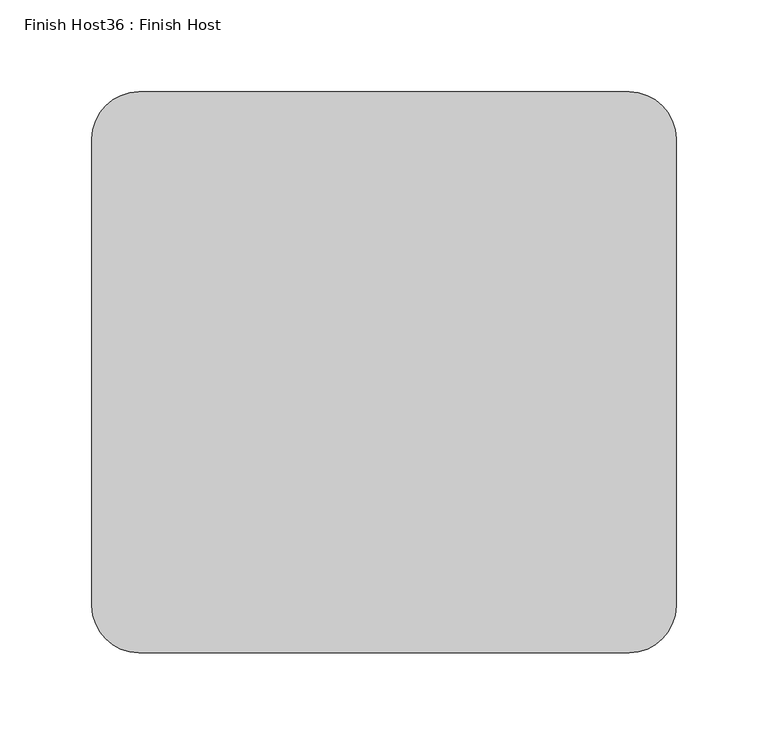
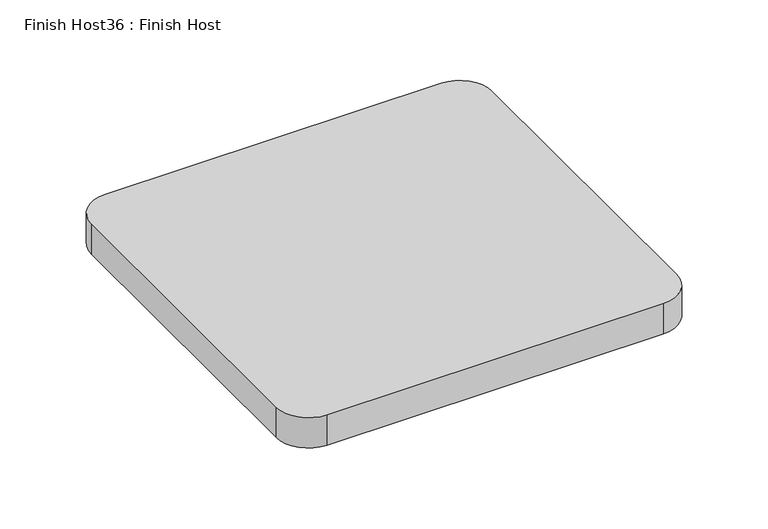
"""IFC4 building model written with IfcOpenShell, lengths in millimetres: proxy geometry, Finish Host36 : Finish Host."""

import ifcopenshell
import ifcopenshell.guid

model = None  # the IFC model being written
_history = None  # IfcOwnerHistory: only IFC2X3 demands one
_inside = {}  # id of a spatial element -> (the spatial element, [elements in it])
_under = {}  # id of a project, library or spatial element -> (it, [spatial elements below it])
_declared = {}  # id of a project -> (the project, [libraries it declares])
_typed = {}  # id of a type object -> (the type object, [elements of that type])
_made_of = {}  # id of a material, layer set ... -> (it, [elements and type objects made of it])


def new_model(schema):
    """Start an empty IFC model of exactly this schema.

    Asked for "IFC4X3", IfcOpenShell would pick the latest addendum, in which some entities
    have other attributes; the version numbers below select the first issue.
    IFC2X3 requires an IfcOwnerHistory on every rooted entity: one is made here for all.
    """
    global model, _history
    if schema == "IFC4X3":
        model = ifcopenshell.file(schema_version=(4, 3, 0, 0))
    else:
        model = ifcopenshell.file(schema=schema)
    _inside.clear()
    _under.clear()
    _declared.clear()
    _typed.clear()
    _made_of.clear()
    _history = None
    if model.schema == "IFC2X3":
        org = make("IfcOrganization", Name="unknown")
        user = make(
            "IfcPersonAndOrganization",
            ThePerson=make("IfcPerson", FamilyName="unknown"),
            TheOrganization=org,
        )
        app = make(
            "IfcApplication",
            ApplicationDeveloper=org,
            Version="unknown",
            ApplicationFullName="unknown",
            ApplicationIdentifier="unknown",
        )
        _history = make(
            "IfcOwnerHistory",
            OwningUser=user,
            OwningApplication=app,
            ChangeAction="ADDED",
            CreationDate=0,
        )
    return model


def make(cls, **values):
    """One entity of the class cls with the attributes given. An attribute that is None is left unset."""
    return model.create_entity(
        cls, **{name: value for name, value in values.items() if value is not None}
    )


def rooted(cls, **values):
    """An entity with a GlobalId (a new one), such as an element, a storey or a relation."""
    return make(cls, GlobalId=ifcopenshell.guid.new(), OwnerHistory=_history, **values)


def si_unit(unit_type, name, prefix=None):
    """IfcSIUnit, for example si_unit("LENGTHUNIT", "METRE", prefix="MILLI")."""
    return make("IfcSIUnit", UnitType=unit_type, Prefix=prefix, Name=name)


def assignment(units):
    """IfcUnitAssignment: the units of a project."""
    return None if units is None else make("IfcUnitAssignment", Units=units)


def point(xyz):
    """IfcCartesianPoint."""
    return None if xyz is None else make("IfcCartesianPoint", Coordinates=xyz)


def direction(xyz):
    """IfcDirection."""
    return None if xyz is None else make("IfcDirection", DirectionRatios=xyz)


def frame(location, z_axis=None, x_axis=None):
    """IfcAxis2Placement3D, a coordinate frame: its origin and axes. An axis left out is left unset."""
    return make(
        "IfcAxis2Placement3D",
        Location=point(location),
        Axis=direction(z_axis),
        RefDirection=direction(x_axis),
    )


def frame_2d(location, x_axis=None):
    """IfcAxis2Placement2D, a coordinate frame in the plane: its origin and x axis."""
    return make(
        "IfcAxis2Placement2D", Location=point(location), RefDirection=direction(x_axis)
    )


def origin():
    """The frame at (0, 0, 0) with its axes left unset."""
    return frame((0.0, 0.0, 0.0))


def origin_with_axes():
    """The frame at (0, 0, 0) with the z axis (0, 0, 1) and the x axis (1, 0, 0) written out."""
    return frame((0.0, 0.0, 0.0), z_axis=(0.0, 0.0, 1.0), x_axis=(1.0, 0.0, 0.0))


def place(relative_to, where):
    """IfcLocalPlacement: puts the frame where relative to a parent placement (None: the world)."""
    return make(
        "IfcLocalPlacement", PlacementRelTo=relative_to, RelativePlacement=where
    )


def context(
    kind, dimensions, precision=None, world=None, true_north=None, identifier=None
):
    """IfcGeometricRepresentationContext, for example the 3D "Model" context."""
    return make(
        "IfcGeometricRepresentationContext",
        ContextIdentifier=identifier,
        ContextType=kind,
        CoordinateSpaceDimension=dimensions,
        Precision=precision,
        WorldCoordinateSystem=world,
        TrueNorth=true_north,
    )


def project(units=None, contexts=None):
    """IfcProject with its units and contexts."""
    return rooted(
        "IfcProject",
        Name="project",
        RepresentationContexts=contexts,
        UnitsInContext=assignment(units),
    )


def spatial(cls, under=None, at=None, **own):
    """A site, building, storey or space (cls), placed at a placement, below another one or the project."""
    s = rooted(cls, ObjectPlacement=at, **own)
    if under is not None:
        _under.setdefault(under.id(), (under, []))[1].append(s)
    return s


def polyline(points):
    """IfcPolyline through the points."""
    return make("IfcPolyline", Points=[point(p) for p in points])


def circle_curve(where, radius):
    """IfcCircle in the frame where."""
    return make("IfcCircle", Position=where, Radius=radius)


def trimmed(basis, trim1, trim2, sense, master):
    """IfcTrimmedCurve: the piece of a basis curve between two trims."""
    return make(
        "IfcTrimmedCurve",
        BasisCurve=basis,
        Trim1=trim1,
        Trim2=trim2,
        SenseAgreement=sense,
        MasterRepresentation=master,
    )


def segment(curve, same_sense, transition):
    """IfcCompositeCurveSegment."""
    return make(
        "IfcCompositeCurveSegment",
        Transition=transition,
        SameSense=same_sense,
        ParentCurve=curve,
    )


def composite_curve(segments, self_intersect=None):
    """IfcCompositeCurve: segments joined end to end."""
    return make("IfcCompositeCurve", Segments=segments, SelfIntersect=self_intersect)


def outline(outer, holes=None, kind="AREA"):
    """IfcArbitraryClosedProfileDef: a profile drawn as a closed curve; with holes, ...WithVoids."""
    if holes is None:
        return make("IfcArbitraryClosedProfileDef", ProfileType=kind, OuterCurve=outer)
    return make(
        "IfcArbitraryProfileDefWithVoids",
        ProfileType=kind,
        OuterCurve=outer,
        InnerCurves=holes,
    )


def extrude(swept, where, along, depth):
    """IfcExtrudedAreaSolid: the profile swept, set in the frame where, extruded along a direction by depth."""
    return make(
        "IfcExtrudedAreaSolid",
        SweptArea=swept,
        Position=where,
        ExtrudedDirection=direction(along),
        Depth=depth,
    )


def shape(context_of_items, identifier, shape_type, items):
    """IfcShapeRepresentation: the items that make up one representation, for example the "Body"."""
    return make(
        "IfcShapeRepresentation",
        ContextOfItems=context_of_items,
        RepresentationIdentifier=identifier,
        RepresentationType=shape_type,
        Items=items,
    )


def source(mapping_origin, context_of_items, identifier, shape_type, items):
    """IfcRepresentationMap: a shape defined once, which mapped items show again and again."""
    return make(
        "IfcRepresentationMap",
        MappingOrigin=mapping_origin,
        MappedRepresentation=shape(context_of_items, identifier, shape_type, items),
    )


def transform(
    local_origin,
    x_axis=None,
    y_axis=None,
    z_axis=None,
    scale=None,
    scale2=None,
    scale3=None,
    uniform=True,
):
    """IfcCartesianTransformationOperator3D, or its non-uniform kind. x_axis, y_axis, z_axis: its Axis1, 2, 3."""
    if uniform:
        return make(
            "IfcCartesianTransformationOperator3D",
            Axis1=direction(x_axis),
            Axis2=direction(y_axis),
            LocalOrigin=point(local_origin),
            Scale=scale,
            Axis3=direction(z_axis),
        )
    return make(
        "IfcCartesianTransformationOperator3DnonUniform",
        Axis1=direction(x_axis),
        Axis2=direction(y_axis),
        LocalOrigin=point(local_origin),
        Scale=scale,
        Axis3=direction(z_axis),
        Scale2=scale2,
        Scale3=scale3,
    )


def mapped(mapping_source, mapping_target):
    """IfcMappedItem: shows the shape of a source again, moved by a transform."""
    return make(
        "IfcMappedItem", MappingSource=mapping_source, MappingTarget=mapping_target
    )


def made_of(thing, what):
    """Note that an element or type object is made of a material, layer set ...; save() writes the relation."""
    if what is not None:
        _made_of.setdefault(what.id(), (what, []))[1].append(thing)
    return thing


def element(
    cls,
    number,
    at=None,
    inside=None,
    cuts=None,
    type_object=None,
    material=None,
    context=None,
    identifier="Body",
    shape_type=None,
    held_by="IfcProductDefinitionShape",
    body=None,
    shapes=None,
    **own,
):
    """One element of the class cls, such as IfcWall. Its Tag is "e" and its number.

    at: its placement. inside: the storey or other place that contains it. cuts: it is an
    opening in that element (IfcRelVoidsElement). A single representation is given by context,
    identifier, shape_type and body (its items); several are given by shapes. held_by: the class
    of the entity that holds the representations. save() writes the other relations.
    """
    e = rooted(cls, Tag="e%d" % number, ObjectPlacement=at, **own)
    if body is not None:
        shapes = [shape(context, identifier, shape_type, body)]
    if shapes is not None:
        e.Representation = make(held_by, Representations=shapes)
    if inside is not None:
        _inside.setdefault(inside.id(), (inside, []))[1].append(e)
    if cuts is not None:
        rooted(
            "IfcRelVoidsElement", RelatingBuildingElement=cuts, RelatedOpeningElement=e
        )
    if type_object is not None:
        _typed.setdefault(type_object.id(), (type_object, []))[1].append(e)
    return made_of(e, material)


def aggregate(whole, parts):
    """IfcRelAggregates: a whole, such as a stair, and the parts it consists of."""
    return rooted("IfcRelAggregates", RelatingObject=whole, RelatedObjects=parts)


def save(model, path):
    """Write the relations noted so far, then the file.

    IfcRelAggregates (storeys below a building ...), IfcRelContainedInSpatialStructure (elements
    in a storey), IfcRelDefinesByType, IfcRelAssociatesMaterial and IfcRelDeclares: one each for
    every whole, place, type object, material and project.
    """
    for whole, parts in _under.values():
        aggregate(whole, parts)
    for where, things in _inside.values():
        rooted(
            "IfcRelContainedInSpatialStructure",
            RelatedElements=things,
            RelatingStructure=where,
        )
    for kind, things in _typed.values():
        rooted("IfcRelDefinesByType", RelatedObjects=things, RelatingType=kind)
    for what, things in _made_of.values():
        rooted("IfcRelAssociatesMaterial", RelatedObjects=things, RelatingMaterial=what)
    for by, libraries in _declared.values():
        rooted("IfcRelDeclares", RelatingContext=by, RelatedDefinitions=libraries)
    model.write(path)


def finish_host36_finish_host_162764ce(model_context):
    return source(origin(), model_context, "Body", "SweptSolid", [
        extrude(outline(composite_curve([segment(polyline([(-54.2342816, 4249.8159302), (-54.2342816, 4503.8159302)]), True, "CONTINUOUS"), segment(trimmed(circle_curve(frame_2d((-28.8342816, 4503.8159302)), 25.4), [point((-54.2342816, 4503.8159302))], [point((-28.8342816, 4529.2159302))], False, "CARTESIAN"), True, "CONTINUOUS"), segment(polyline([(-28.8342816, 4529.2159302), (237.8657184, 4529.2159302)]), True, "CONTINUOUS"), segment(trimmed(circle_curve(frame_2d((237.8657184, 4503.8159302)), 25.4), [point((237.8657184, 4529.2159302))], [point((263.2657184, 4503.8159302))], False, "CARTESIAN"), True, "CONTINUOUS"), segment(polyline([(263.2657184, 4503.8159302), (263.2657184, 4249.8159302)]), True, "CONTINUOUS"), segment(trimmed(circle_curve(frame_2d((237.8657184, 4249.8159302)), 25.4), [point((263.2657184, 4249.8159302))], [point((237.8657184, 4224.4159302))], False, "CARTESIAN"), True, "CONTINUOUS"), segment(polyline([(237.8657184, 4224.4159302), (-28.8342816, 4224.4159302)]), True, "CONTINUOUS"), segment(trimmed(circle_curve(frame_2d((-28.8342816, 4249.8159302)), 25.4), [point((-28.8342816, 4224.4159302))], [point((-54.2342816, 4249.8159302))], False, "CARTESIAN"), True, "CONTINUOUS")], self_intersect=False)), origin_with_axes(), (0.0, 0.0, 1.0), 25.4),
    ])


if __name__ == "__main__":
    model = new_model("IFC4")
    model_context = context("Model", 3, world=origin())
    ifc_project = project(units=[si_unit("LENGTHUNIT", "METRE", prefix="MILLI")], contexts=[model_context])
    site = spatial("IfcSite", under=ifc_project)
    building = spatial("IfcBuilding", under=site)
    placement = place(None, origin())
    finish_host36_finish_host_shape = finish_host36_finish_host_162764ce(model_context)
    element("IfcBuildingElementProxy", 1, Name="Finish Host36 : Finish Host", ObjectType="Finish Host36 : Finish Host", at=placement, inside=building, context=model_context, shape_type="MappedRepresentation", body=[
        mapped(finish_host36_finish_host_shape, transform((0.0, 0.0, 0.0), x_axis=(1.0, 0.0, 0.0), y_axis=(0.0, 1.0, 0.0), z_axis=(0.0, 0.0, 1.0))),
    ])
    save(model, "model.ifc")

# Revit data of these elements
# Type "Finish Host36 : Finish Host"
#   Countertop Material = Fabric - Teknion - S144 - Synaptic - Axon
# Element 1 (IfcBuildingElementProxy, "Finish Host36 : Finish Host")
#   Materials on its faces: "Fabric - Teknion - S144 - Synaptic - Axon"
# Materials
#   "Fabric - Teknion - S144 - Synaptic - Axon": class "Fabric", colour RGB 22 20 20, transparency 0, Model = "S144", Manufacturer = "Teknion Studio", URL = "http://www.teknionstudio.com/", Description = "Axon Synaptic", Cost = 0
